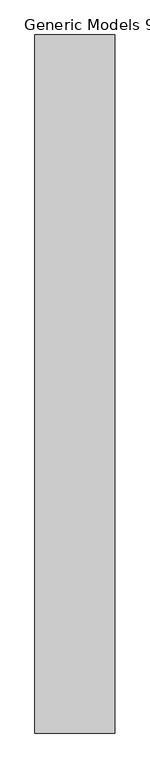
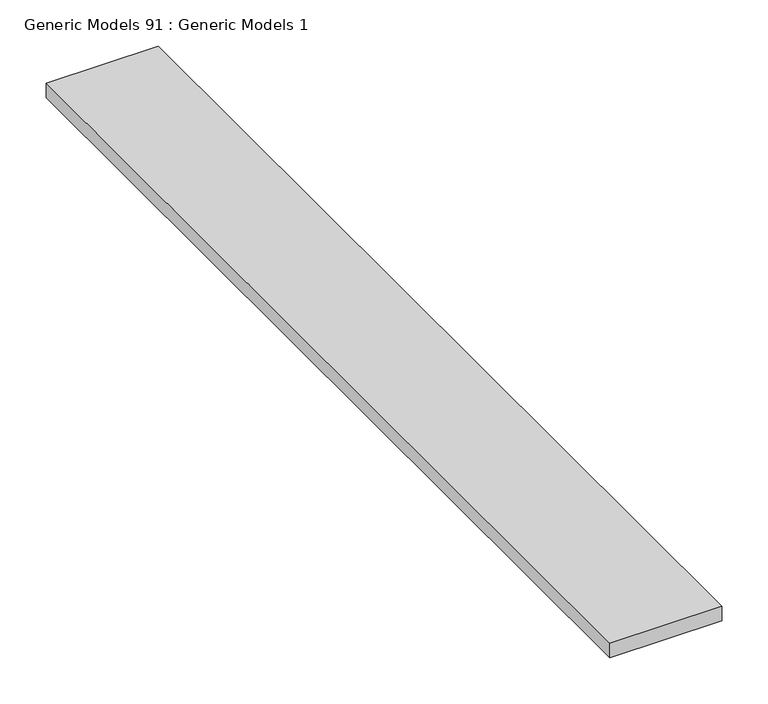
"""IFC4 building model written with IfcOpenShell, lengths in millimetres: proxy geometry, Generic Models 91 : Generic Models 1."""

from ifc_helpers import new_model, si_unit, frame, origin, place, context, project, spatial, polyline, outline, extrude, source, transform, mapped, element, save


def generic_models_91_generic_models_1_c80baf30(model_context):
    return source(origin(), model_context, "Body", "SweptSolid", [
        extrude(outline(polyline([(45764.2985531, 0.0), (45624.5985531, 0.0), (45624.5985531, 1219.2), (45764.2985531, 1219.2), (45764.2985531, 0.0)])), frame((0.0, 0.0, 2250.523933), z_axis=(0.0, 0.0, 1.0), x_axis=(1.0, 0.0, 0.0)), (0.0, 0.0, 1.0), 19.05),
    ])


if __name__ == "__main__":
    model = new_model("IFC4")
    model_context = context("Model", 3, world=origin())
    ifc_project = project(units=[si_unit("LENGTHUNIT", "METRE", prefix="MILLI")], contexts=[model_context])
    site = spatial("IfcSite", under=ifc_project)
    building = spatial("IfcBuilding", under=site)
    placement = place(None, origin())
    generic_models_91_generic_models_1_shape = generic_models_91_generic_models_1_c80baf30(model_context)
    element("IfcBuildingElementProxy", 1, Name="Generic Models 91 : Generic Models 1", ObjectType="Generic Models 91 : Generic Models 1", at=placement, inside=building, context=model_context, shape_type="MappedRepresentation", body=[
        mapped(generic_models_91_generic_models_1_shape, transform((0.0, 0.0, 0.0), x_axis=(1.0, 0.0, 0.0), y_axis=(0.0, 1.0, 0.0), z_axis=(0.0, 0.0, 1.0))),
    ])
    save(model, "model.ifc")

# Revit data of these elements
# Element 1 (IfcBuildingElementProxy, "Generic Models 91 : Generic Models 1")
#   Materials on its faces: "STAINED WOOD TRIM TO MATCH EXISTING"
# Materials
#   "STAINED WOOD TRIM TO MATCH EXISTING": class "Wood", colour RGB 144 113 62, transparency 0, Description = "Pinus Echinata", Cost = 0
